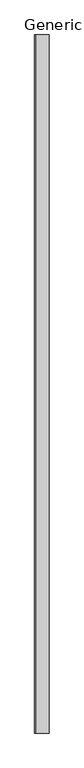
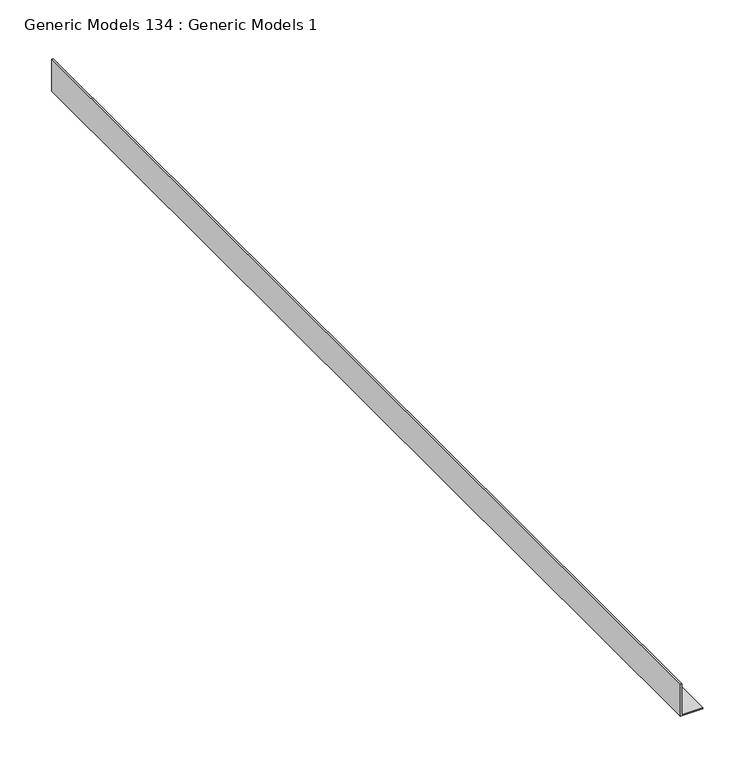
"""IFC4 building model written with IfcOpenShell, lengths in millimetres: proxy geometry, Generic Models 134 : Generic Models 1."""

import ifcopenshell
import ifcopenshell.guid

model = None  # the IFC model being written
_history = None  # IfcOwnerHistory: only IFC2X3 demands one
_inside = {}  # id of a spatial element -> (the spatial element, [elements in it])
_under = {}  # id of a project, library or spatial element -> (it, [spatial elements below it])
_declared = {}  # id of a project -> (the project, [libraries it declares])
_typed = {}  # id of a type object -> (the type object, [elements of that type])
_made_of = {}  # id of a material, layer set ... -> (it, [elements and type objects made of it])


def new_model(schema):
    """Start an empty IFC model of exactly this schema.

    Asked for "IFC4X3", IfcOpenShell would pick the latest addendum, in which some entities
    have other attributes; the version numbers below select the first issue.
    IFC2X3 requires an IfcOwnerHistory on every rooted entity: one is made here for all.
    """
    global model, _history
    if schema == "IFC4X3":
        model = ifcopenshell.file(schema_version=(4, 3, 0, 0))
    else:
        model = ifcopenshell.file(schema=schema)
    _inside.clear()
    _under.clear()
    _declared.clear()
    _typed.clear()
    _made_of.clear()
    _history = None
    if model.schema == "IFC2X3":
        org = make("IfcOrganization", Name="unknown")
        user = make(
            "IfcPersonAndOrganization",
            ThePerson=make("IfcPerson", FamilyName="unknown"),
            TheOrganization=org,
        )
        app = make(
            "IfcApplication",
            ApplicationDeveloper=org,
            Version="unknown",
            ApplicationFullName="unknown",
            ApplicationIdentifier="unknown",
        )
        _history = make(
            "IfcOwnerHistory",
            OwningUser=user,
            OwningApplication=app,
            ChangeAction="ADDED",
            CreationDate=0,
        )
    return model


def make(cls, **values):
    """One entity of the class cls with the attributes given. An attribute that is None is left unset."""
    return model.create_entity(
        cls, **{name: value for name, value in values.items() if value is not None}
    )


def rooted(cls, **values):
    """An entity with a GlobalId (a new one), such as an element, a storey or a relation."""
    return make(cls, GlobalId=ifcopenshell.guid.new(), OwnerHistory=_history, **values)


def si_unit(unit_type, name, prefix=None):
    """IfcSIUnit, for example si_unit("LENGTHUNIT", "METRE", prefix="MILLI")."""
    return make("IfcSIUnit", UnitType=unit_type, Prefix=prefix, Name=name)


def assignment(units):
    """IfcUnitAssignment: the units of a project."""
    return None if units is None else make("IfcUnitAssignment", Units=units)


def point(xyz):
    """IfcCartesianPoint."""
    return None if xyz is None else make("IfcCartesianPoint", Coordinates=xyz)


def direction(xyz):
    """IfcDirection."""
    return None if xyz is None else make("IfcDirection", DirectionRatios=xyz)


def frame(location, z_axis=None, x_axis=None):
    """IfcAxis2Placement3D, a coordinate frame: its origin and axes. An axis left out is left unset."""
    return make(
        "IfcAxis2Placement3D",
        Location=point(location),
        Axis=direction(z_axis),
        RefDirection=direction(x_axis),
    )


def origin():
    """The frame at (0, 0, 0) with its axes left unset."""
    return frame((0.0, 0.0, 0.0))


def place(relative_to, where):
    """IfcLocalPlacement: puts the frame where relative to a parent placement (None: the world)."""
    return make(
        "IfcLocalPlacement", PlacementRelTo=relative_to, RelativePlacement=where
    )


def context(
    kind, dimensions, precision=None, world=None, true_north=None, identifier=None
):
    """IfcGeometricRepresentationContext, for example the 3D "Model" context."""
    return make(
        "IfcGeometricRepresentationContext",
        ContextIdentifier=identifier,
        ContextType=kind,
        CoordinateSpaceDimension=dimensions,
        Precision=precision,
        WorldCoordinateSystem=world,
        TrueNorth=true_north,
    )


def project(units=None, contexts=None):
    """IfcProject with its units and contexts."""
    return rooted(
        "IfcProject",
        Name="project",
        RepresentationContexts=contexts,
        UnitsInContext=assignment(units),
    )


def spatial(cls, under=None, at=None, **own):
    """A site, building, storey or space (cls), placed at a placement, below another one or the project."""
    s = rooted(cls, ObjectPlacement=at, **own)
    if under is not None:
        _under.setdefault(under.id(), (under, []))[1].append(s)
    return s


def polyline(points):
    """IfcPolyline through the points."""
    return make("IfcPolyline", Points=[point(p) for p in points])


def outline(outer, holes=None, kind="AREA"):
    """IfcArbitraryClosedProfileDef: a profile drawn as a closed curve; with holes, ...WithVoids."""
    if holes is None:
        return make("IfcArbitraryClosedProfileDef", ProfileType=kind, OuterCurve=outer)
    return make(
        "IfcArbitraryProfileDefWithVoids",
        ProfileType=kind,
        OuterCurve=outer,
        InnerCurves=holes,
    )


def extrude(swept, where, along, depth):
    """IfcExtrudedAreaSolid: the profile swept, set in the frame where, extruded along a direction by depth."""
    return make(
        "IfcExtrudedAreaSolid",
        SweptArea=swept,
        Position=where,
        ExtrudedDirection=direction(along),
        Depth=depth,
    )


def shape(context_of_items, identifier, shape_type, items):
    """IfcShapeRepresentation: the items that make up one representation, for example the "Body"."""
    return make(
        "IfcShapeRepresentation",
        ContextOfItems=context_of_items,
        RepresentationIdentifier=identifier,
        RepresentationType=shape_type,
        Items=items,
    )


def source(mapping_origin, context_of_items, identifier, shape_type, items):
    """IfcRepresentationMap: a shape defined once, which mapped items show again and again."""
    return make(
        "IfcRepresentationMap",
        MappingOrigin=mapping_origin,
        MappedRepresentation=shape(context_of_items, identifier, shape_type, items),
    )


def transform(
    local_origin,
    x_axis=None,
    y_axis=None,
    z_axis=None,
    scale=None,
    scale2=None,
    scale3=None,
    uniform=True,
):
    """IfcCartesianTransformationOperator3D, or its non-uniform kind. x_axis, y_axis, z_axis: its Axis1, 2, 3."""
    if uniform:
        return make(
            "IfcCartesianTransformationOperator3D",
            Axis1=direction(x_axis),
            Axis2=direction(y_axis),
            LocalOrigin=point(local_origin),
            Scale=scale,
            Axis3=direction(z_axis),
        )
    return make(
        "IfcCartesianTransformationOperator3DnonUniform",
        Axis1=direction(x_axis),
        Axis2=direction(y_axis),
        LocalOrigin=point(local_origin),
        Scale=scale,
        Axis3=direction(z_axis),
        Scale2=scale2,
        Scale3=scale3,
    )


def mapped(mapping_source, mapping_target):
    """IfcMappedItem: shows the shape of a source again, moved by a transform."""
    return make(
        "IfcMappedItem", MappingSource=mapping_source, MappingTarget=mapping_target
    )


def made_of(thing, what):
    """Note that an element or type object is made of a material, layer set ...; save() writes the relation."""
    if what is not None:
        _made_of.setdefault(what.id(), (what, []))[1].append(thing)
    return thing


def element(
    cls,
    number,
    at=None,
    inside=None,
    cuts=None,
    type_object=None,
    material=None,
    context=None,
    identifier="Body",
    shape_type=None,
    held_by="IfcProductDefinitionShape",
    body=None,
    shapes=None,
    **own,
):
    """One element of the class cls, such as IfcWall. Its Tag is "e" and its number.

    at: its placement. inside: the storey or other place that contains it. cuts: it is an
    opening in that element (IfcRelVoidsElement). A single representation is given by context,
    identifier, shape_type and body (its items); several are given by shapes. held_by: the class
    of the entity that holds the representations. save() writes the other relations.
    """
    e = rooted(cls, Tag="e%d" % number, ObjectPlacement=at, **own)
    if body is not None:
        shapes = [shape(context, identifier, shape_type, body)]
    if shapes is not None:
        e.Representation = make(held_by, Representations=shapes)
    if inside is not None:
        _inside.setdefault(inside.id(), (inside, []))[1].append(e)
    if cuts is not None:
        rooted(
            "IfcRelVoidsElement", RelatingBuildingElement=cuts, RelatedOpeningElement=e
        )
    if type_object is not None:
        _typed.setdefault(type_object.id(), (type_object, []))[1].append(e)
    return made_of(e, material)


def aggregate(whole, parts):
    """IfcRelAggregates: a whole, such as a stair, and the parts it consists of."""
    return rooted("IfcRelAggregates", RelatingObject=whole, RelatedObjects=parts)


def save(model, path):
    """Write the relations noted so far, then the file.

    IfcRelAggregates (storeys below a building ...), IfcRelContainedInSpatialStructure (elements
    in a storey), IfcRelDefinesByType, IfcRelAssociatesMaterial and IfcRelDeclares: one each for
    every whole, place, type object, material and project.
    """
    for whole, parts in _under.values():
        aggregate(whole, parts)
    for where, things in _inside.values():
        rooted(
            "IfcRelContainedInSpatialStructure",
            RelatedElements=things,
            RelatingStructure=where,
        )
    for kind, things in _typed.values():
        rooted("IfcRelDefinesByType", RelatedObjects=things, RelatingType=kind)
    for what, things in _made_of.values():
        rooted("IfcRelAssociatesMaterial", RelatedObjects=things, RelatingMaterial=what)
    for by, libraries in _declared.values():
        rooted("IfcRelDeclares", RelatingContext=by, RelatedDefinitions=libraries)
    model.write(path)


def generic_models_134_generic_models_1_881594d0(model_context):
    return source(origin(), model_context, "Body", "SweptSolid", [
        extrude(outline(polyline([(2051.1444308, 46951.7485531), (2013.0444308, 46951.7485531), (2013.0444308, 46977.1485531), (2014.6319308, 46977.1485531), (2014.6319308, 46953.3360531), (2051.1444308, 46953.3360531), (2051.1444308, 46951.7485531)])), frame((0.0, 0.0, 0.0), z_axis=(0.0, 1.0, 0.0), x_axis=(0.0, 0.0, 1.0)), (0.0, 0.0, 1.0), 1219.2),
    ])


if __name__ == "__main__":
    model = new_model("IFC4")
    model_context = context("Model", 3, world=origin())
    ifc_project = project(units=[si_unit("LENGTHUNIT", "METRE", prefix="MILLI")], contexts=[model_context])
    site = spatial("IfcSite", under=ifc_project)
    building = spatial("IfcBuilding", under=site)
    placement = place(None, origin())
    generic_models_134_generic_models_1_shape = generic_models_134_generic_models_1_881594d0(model_context)
    element("IfcBuildingElementProxy", 1, Name="Generic Models 134 : Generic Models 1", ObjectType="Generic Models 134 : Generic Models 1", at=placement, inside=building, context=model_context, shape_type="MappedRepresentation", body=[
        mapped(generic_models_134_generic_models_1_shape, transform((0.0, 0.0, 0.0), x_axis=(1.0, 0.0, 0.0), y_axis=(0.0, 1.0, 0.0), z_axis=(0.0, 0.0, 1.0))),
    ])
    save(model, "model.ifc")

# Revit data of these elements
# Element 1 (IfcBuildingElementProxy, "Generic Models 134 : Generic Models 1")
#   Materials on its faces: "CEILING TRACK TO MATCH EXISTING"
# Materials
#   "CEILING TRACK TO MATCH EXISTING": class "Unassigned", colour RGB 210 209 208, transparency 0, Keynote = "M05121300.02", Cost = 0
